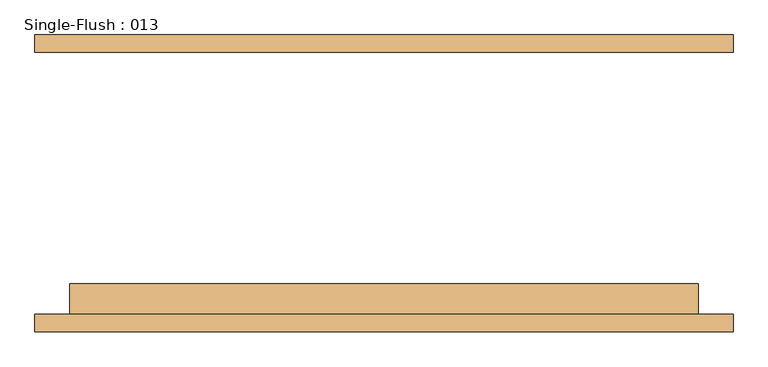
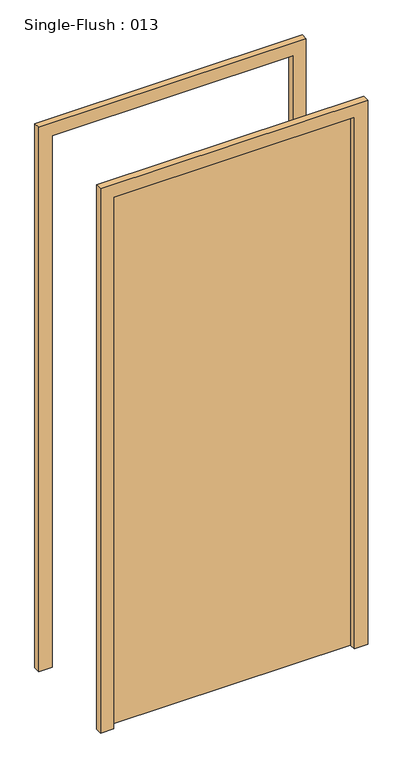
"""IFC4 building model written with IfcOpenShell, lengths in millimetres: door geometry, Single-Flush : 013."""

from ifc_helpers import new_model, si_unit, frame, origin, origin_with_axes, place, context, project, spatial, polyline, outline, extrude, source, transform, mapped, element, save


def single_flush_013_d0afb6d8(model_context):
    return source(origin(), model_context, "Body", "SweptSolid", [
        extrude(outline(polyline([(2184.4, -508.0), (0.0, -508.0), (0.0, -457.2), (2133.6, -457.2), (2133.6, 457.2), (0.0, 457.2), (0.0, 508.0), (2184.4, 508.0), (2184.4, -508.0)])), frame((0.0, -215.9, 0.0), z_axis=(0.0, 1.0, 0.0), x_axis=(0.0, 0.0, 1.0)), (0.0, 0.0, 1.0), 25.4),
        extrude(outline(polyline([(2184.4, 508.0), (2184.4, -508.0), (0.0, -508.0), (0.0, -457.2), (2133.6, -457.2), (2133.6, 457.2), (0.0, 457.2), (0.0, 508.0), (2184.4, 508.0)])), frame((0.0, 190.5, 0.0), z_axis=(0.0, 1.0, 0.0), x_axis=(0.0, 0.0, 1.0)), (0.0, 0.0, 1.0), 25.4),
        extrude(outline(polyline([(457.2, -146.05), (457.2, -190.5), (-457.2, -190.5), (-457.2, -146.05), (457.2, -146.05)])), origin_with_axes(), (0.0, 0.0, 1.0), 2133.6),
    ])


if __name__ == "__main__":
    model = new_model("IFC4")
    model_context = context("Model", 3, world=origin())
    ifc_project = project(units=[si_unit("LENGTHUNIT", "METRE", prefix="MILLI")], contexts=[model_context])
    site = spatial("IfcSite", under=ifc_project)
    building = spatial("IfcBuilding", under=site)
    placement = place(None, origin())
    single_flush_013_shape = single_flush_013_d0afb6d8(model_context)
    element("IfcDoor", 1, ObjectType="Single-Flush : 013", at=placement, inside=building, context=model_context, shape_type="MappedRepresentation", body=[
        mapped(single_flush_013_shape, transform((0.0, 0.0, 0.0), x_axis=(1.0, 0.0, 0.0), y_axis=(0.0, 1.0, 0.0), z_axis=(0.0, 0.0, 1.0))),
    ])
    save(model, "model.ifc")

# Revit data of these elements
# Type "Single-Flush : 013"
#   Type Mark = "013"
#   Construction Type Id = "MDOOR"
#   Assembly Code = "C1020"
#   Analytic Construction = "Metal"
#   Thickness = 0' - 1 3/4"
#   Heat Transfer Coefficient (U) = 3.7021 W/(m²·K)
#   Height = 7' - 0"
#   Trim Projection Ext = 0' - 1"
#   Trim Projection Int = 0' - 1"
#   Trim Width = 0' - 2"
#   Width = 3' - 0"
#   Door Material = 05 - Metal - Steel
#   Frame Material = 05 - Metal - Aluminum
#   Visual Light Transmittance = 0
#   Solar Heat Gain Coefficient = 0
#   Function = (empty or 0)
#   Wall Closure = (empty or 0)
# Element 1 (IfcDoor, "Single-Flush : 013")
#   Materials on its faces: "05 - Metal - Aluminum", "05 - Metal - Steel"
# Materials
#   "05 - Metal - Steel": class "Unassigned", colour RGB 199 199 199, transparency 0, Description = "Steel"
#   "05 - Metal - Aluminum": class "Unassigned", colour RGB 247 247 247, transparency 0, Description = "Aluminum"
